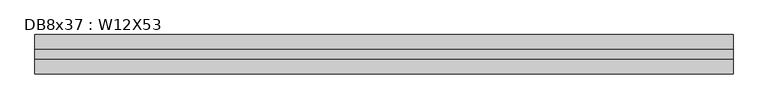
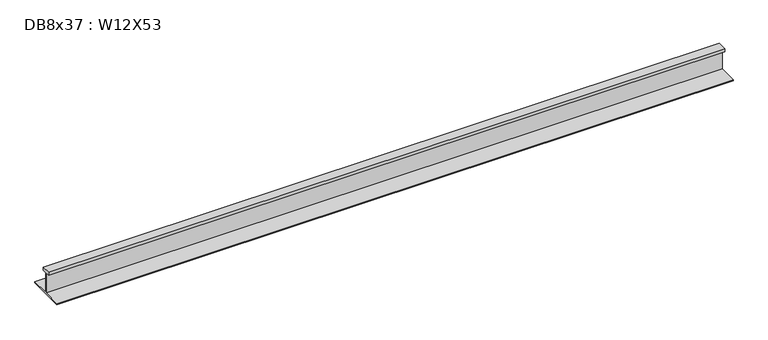
"""IFC4 building model written with IfcOpenShell, lengths in millimetres: beam geometry, DB8x37 : W12X53."""

from ifc_helpers import new_model, si_unit, frame, origin, place, context, project, spatial, polyline, outline, extrude, source, transform, mapped, element, save


def db8x37_w12x53_31252158(model_context):
    return source(origin(), model_context, "Body", "SweptSolid", [
        extrude(outline(polyline([(38.1, 145.415), (38.1, 120.015), (2.921, 120.015), (2.921, -48.4505), (152.4, -48.4505), (152.4, -58.1025), (-152.4, -58.1025), (-152.4, -48.4505), (-2.921, -48.4505), (-2.921, 120.015), (-38.1, 120.015), (-38.1, 145.415), (38.1, 145.415)])), frame((-2708.529, 0.0, 0.0), z_axis=(1.0, 0.0, 0.0), x_axis=(0.0, 1.0, 0.0)), (0.0, 0.0, 1.0), 5414.645),
    ])


if __name__ == "__main__":
    model = new_model("IFC4")
    model_context = context("Model", 3, world=origin())
    ifc_project = project(units=[si_unit("LENGTHUNIT", "METRE", prefix="MILLI")], contexts=[model_context])
    site = spatial("IfcSite", under=ifc_project)
    building = spatial("IfcBuilding", under=site)
    placement = place(None, origin())
    db8x37_w12x53_shape = db8x37_w12x53_31252158(model_context)
    element("IfcBeam", 1, ObjectType="DB8x37 : W12X53", at=placement, inside=building, context=model_context, shape_type="MappedRepresentation", body=[
        mapped(db8x37_w12x53_shape, transform((0.0, 0.0, 0.0), x_axis=(1.0, 0.0, 0.0), y_axis=(0.0, 1.0, 0.0), z_axis=(0.0, 0.0, 1.0))),
    ])
    save(model, "model.ifc")

# Revit data of these elements
# Type "DB8x37 : W12X53"
#   Assembly Code = "B10"
#   W = 53
#   Length [instance default] = 5' - 0"
#   bf = 0' - 10"
#   d = 1' - 0.1"
#   k = 0' - 1 3/8"
#   k2 = 0' - 0.8"
#   tf = 0' - 0.575"
#   tw = 0' - 0.345"
#   A = 0.108333 SF
#   Structural Material [instance default] = Steel ASTM A992
# Element 1 (IfcBeam, "DB8x37 : W12X53")
#   Materials on its faces: "Steel ASTM A992"
# Materials
#   "Steel ASTM A992": class "Metal", colour RGB 199 199 199, transparency 0, Description = "Structural steel 50ksi", Cost = 0
